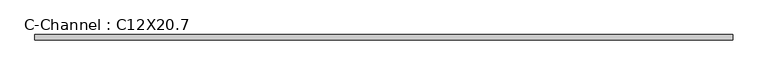
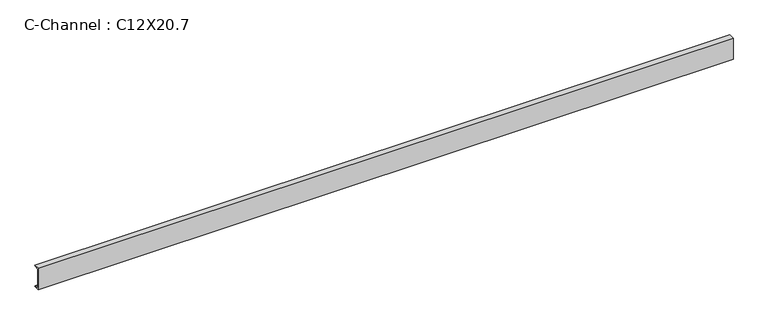
"""IFC4 building model written with IfcOpenShell, lengths in millimetres: beam geometry, C-Channel : C12X20.7."""

from ifc_helpers import new_model, si_unit, point, frame, frame_2d, origin, place, context, project, spatial, polyline, circle_curve, trimmed, segment, composite_curve, outline, extrude, source, transform, mapped, element, save


def c_channel_c12x20_7_eb780fe2(model_context):
    return source(origin(), model_context, "Body", "SweptSolid", [
        extrude(outline(composite_curve([segment(polyline([(-17.7292, 152.4), (56.9468, 152.4)]), True, "CONTINUOUS"), segment(trimmed(circle_curve(frame_2d((44.2214, 152.4)), 12.7254), [point((56.9468, 152.4))], [point((44.2214, 139.6746))], False, "CARTESIAN"), True, "CONTINUOUS"), segment(polyline([(44.2214, 139.6746), (-10.5664, 130.997065), (-10.5664, -130.997065), (44.2214, -139.6746)]), True, "CONTINUOUS"), segment(trimmed(circle_curve(frame_2d((44.2214, -152.4)), 12.7254), [point((44.2214, -139.6746))], [point((56.9468, -152.4))], False, "CARTESIAN"), True, "CONTINUOUS"), segment(polyline([(56.9468, -152.4), (-17.7292, -152.4), (-17.7292, 152.4)]), True, "CONTINUOUS")], self_intersect=False)), frame((-4975.4737258, 0.0, 0.0), z_axis=(1.0, 0.0, 0.0), x_axis=(0.0, 1.0, 0.0)), (0.0, 0.0, 1.0), 9379.994427),
    ])


if __name__ == "__main__":
    model = new_model("IFC4")
    model_context = context("Model", 3, world=origin())
    ifc_project = project(units=[si_unit("LENGTHUNIT", "METRE", prefix="MILLI")], contexts=[model_context])
    site = spatial("IfcSite", under=ifc_project)
    building = spatial("IfcBuilding", under=site)
    placement = place(None, origin())
    c_channel_c12x20_7_shape = c_channel_c12x20_7_eb780fe2(model_context)
    element("IfcBeam", 1, ObjectType="C-Channel : C12X20.7", at=placement, inside=building, context=model_context, shape_type="MappedRepresentation", body=[
        mapped(c_channel_c12x20_7_shape, transform((0.0, 0.0, 0.0), x_axis=(1.0, 0.0, 0.0), y_axis=(0.0, 1.0, 0.0), z_axis=(0.0, 0.0, 1.0))),
    ])
    save(model, "model.ifc")

# Revit data of these elements
# Type "C-Channel : C12X20.7"
#   Assembly Code = "B10"
#   W = 20.7
#   Start Extension Calculation [instance default] = 10' - 0"
#   Start Extension [instance default] = -0' - 0 1/2"
#   End Extension Calculation [instance default] = 10' - 0"
#   End Extension [instance default] = -0' - 0 1/2"
#   Length [instance default] = 5' - 0"
#   bf = 0' - 2.94"
#   d = 1' - 0"
#   tf = 0' - 0.501"
#   tw = 0' - 0.282"
#   x = 0' - 0.698"
#   A = 0.0422222 SF
#   Structural Material [instance default] = Metal - Steel - ASTM A36
# Element 1 (IfcBeam, "C-Channel : C12X20.7")
#   Materials on its faces: "Metal - Steel - ASTM A36"
# Materials
#   "Metal - Steel - ASTM A36": class "Metal", colour RGB 199 199 199, transparency 0
